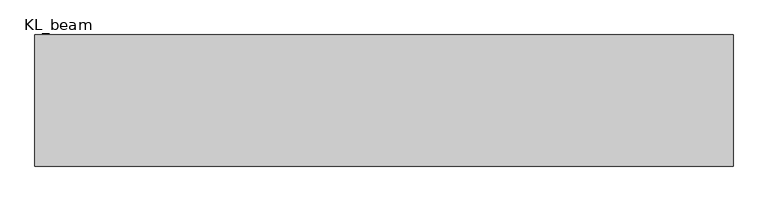
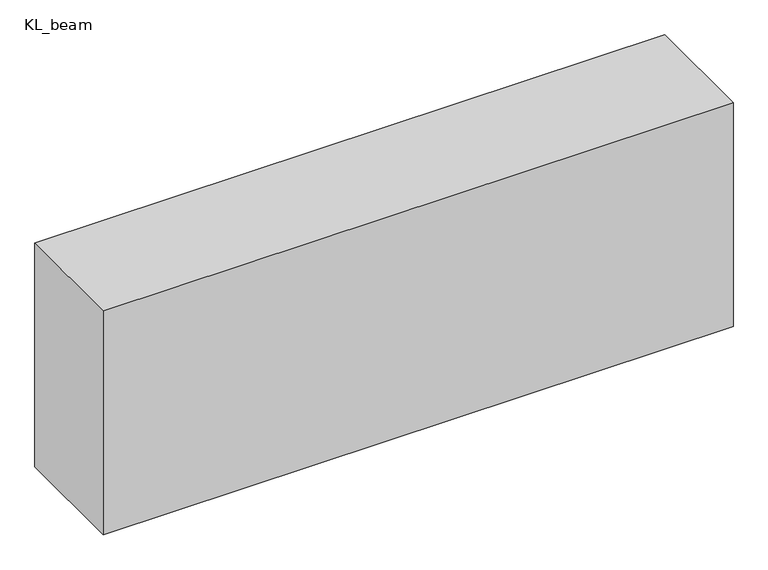
"""IFC4 building model written with IfcOpenShell, lengths in millimetres: beam geometry, 混凝土 - 矩形梁 : KL_beam."""

import ifcopenshell
import ifcopenshell.guid

model = None  # the IFC model being written
_history = None  # IfcOwnerHistory: only IFC2X3 demands one
_inside = {}  # id of a spatial element -> (the spatial element, [elements in it])
_under = {}  # id of a project, library or spatial element -> (it, [spatial elements below it])
_declared = {}  # id of a project -> (the project, [libraries it declares])
_typed = {}  # id of a type object -> (the type object, [elements of that type])
_made_of = {}  # id of a material, layer set ... -> (it, [elements and type objects made of it])


def new_model(schema):
    """Start an empty IFC model of exactly this schema.

    Asked for "IFC4X3", IfcOpenShell would pick the latest addendum, in which some entities
    have other attributes; the version numbers below select the first issue.
    IFC2X3 requires an IfcOwnerHistory on every rooted entity: one is made here for all.
    """
    global model, _history
    if schema == "IFC4X3":
        model = ifcopenshell.file(schema_version=(4, 3, 0, 0))
    else:
        model = ifcopenshell.file(schema=schema)
    _inside.clear()
    _under.clear()
    _declared.clear()
    _typed.clear()
    _made_of.clear()
    _history = None
    if model.schema == "IFC2X3":
        org = make("IfcOrganization", Name="unknown")
        user = make(
            "IfcPersonAndOrganization",
            ThePerson=make("IfcPerson", FamilyName="unknown"),
            TheOrganization=org,
        )
        app = make(
            "IfcApplication",
            ApplicationDeveloper=org,
            Version="unknown",
            ApplicationFullName="unknown",
            ApplicationIdentifier="unknown",
        )
        _history = make(
            "IfcOwnerHistory",
            OwningUser=user,
            OwningApplication=app,
            ChangeAction="ADDED",
            CreationDate=0,
        )
    return model


def make(cls, **values):
    """One entity of the class cls with the attributes given. An attribute that is None is left unset."""
    return model.create_entity(
        cls, **{name: value for name, value in values.items() if value is not None}
    )


def rooted(cls, **values):
    """An entity with a GlobalId (a new one), such as an element, a storey or a relation."""
    return make(cls, GlobalId=ifcopenshell.guid.new(), OwnerHistory=_history, **values)


def si_unit(unit_type, name, prefix=None):
    """IfcSIUnit, for example si_unit("LENGTHUNIT", "METRE", prefix="MILLI")."""
    return make("IfcSIUnit", UnitType=unit_type, Prefix=prefix, Name=name)


def assignment(units):
    """IfcUnitAssignment: the units of a project."""
    return None if units is None else make("IfcUnitAssignment", Units=units)


def point(xyz):
    """IfcCartesianPoint."""
    return None if xyz is None else make("IfcCartesianPoint", Coordinates=xyz)


def direction(xyz):
    """IfcDirection."""
    return None if xyz is None else make("IfcDirection", DirectionRatios=xyz)


def frame(location, z_axis=None, x_axis=None):
    """IfcAxis2Placement3D, a coordinate frame: its origin and axes. An axis left out is left unset."""
    return make(
        "IfcAxis2Placement3D",
        Location=point(location),
        Axis=direction(z_axis),
        RefDirection=direction(x_axis),
    )


def origin():
    """The frame at (0, 0, 0) with its axes left unset."""
    return frame((0.0, 0.0, 0.0))


def place(relative_to, where):
    """IfcLocalPlacement: puts the frame where relative to a parent placement (None: the world)."""
    return make(
        "IfcLocalPlacement", PlacementRelTo=relative_to, RelativePlacement=where
    )


def context(
    kind, dimensions, precision=None, world=None, true_north=None, identifier=None
):
    """IfcGeometricRepresentationContext, for example the 3D "Model" context."""
    return make(
        "IfcGeometricRepresentationContext",
        ContextIdentifier=identifier,
        ContextType=kind,
        CoordinateSpaceDimension=dimensions,
        Precision=precision,
        WorldCoordinateSystem=world,
        TrueNorth=true_north,
    )


def project(units=None, contexts=None):
    """IfcProject with its units and contexts."""
    return rooted(
        "IfcProject",
        Name="project",
        RepresentationContexts=contexts,
        UnitsInContext=assignment(units),
    )


def spatial(cls, under=None, at=None, **own):
    """A site, building, storey or space (cls), placed at a placement, below another one or the project."""
    s = rooted(cls, ObjectPlacement=at, **own)
    if under is not None:
        _under.setdefault(under.id(), (under, []))[1].append(s)
    return s


def polyline(points):
    """IfcPolyline through the points."""
    return make("IfcPolyline", Points=[point(p) for p in points])


def outline(outer, holes=None, kind="AREA"):
    """IfcArbitraryClosedProfileDef: a profile drawn as a closed curve; with holes, ...WithVoids."""
    if holes is None:
        return make("IfcArbitraryClosedProfileDef", ProfileType=kind, OuterCurve=outer)
    return make(
        "IfcArbitraryProfileDefWithVoids",
        ProfileType=kind,
        OuterCurve=outer,
        InnerCurves=holes,
    )


def extrude(swept, where, along, depth):
    """IfcExtrudedAreaSolid: the profile swept, set in the frame where, extruded along a direction by depth."""
    return make(
        "IfcExtrudedAreaSolid",
        SweptArea=swept,
        Position=where,
        ExtrudedDirection=direction(along),
        Depth=depth,
    )


def shape(context_of_items, identifier, shape_type, items):
    """IfcShapeRepresentation: the items that make up one representation, for example the "Body"."""
    return make(
        "IfcShapeRepresentation",
        ContextOfItems=context_of_items,
        RepresentationIdentifier=identifier,
        RepresentationType=shape_type,
        Items=items,
    )


def source(mapping_origin, context_of_items, identifier, shape_type, items):
    """IfcRepresentationMap: a shape defined once, which mapped items show again and again."""
    return make(
        "IfcRepresentationMap",
        MappingOrigin=mapping_origin,
        MappedRepresentation=shape(context_of_items, identifier, shape_type, items),
    )


def transform(
    local_origin,
    x_axis=None,
    y_axis=None,
    z_axis=None,
    scale=None,
    scale2=None,
    scale3=None,
    uniform=True,
):
    """IfcCartesianTransformationOperator3D, or its non-uniform kind. x_axis, y_axis, z_axis: its Axis1, 2, 3."""
    if uniform:
        return make(
            "IfcCartesianTransformationOperator3D",
            Axis1=direction(x_axis),
            Axis2=direction(y_axis),
            LocalOrigin=point(local_origin),
            Scale=scale,
            Axis3=direction(z_axis),
        )
    return make(
        "IfcCartesianTransformationOperator3DnonUniform",
        Axis1=direction(x_axis),
        Axis2=direction(y_axis),
        LocalOrigin=point(local_origin),
        Scale=scale,
        Axis3=direction(z_axis),
        Scale2=scale2,
        Scale3=scale3,
    )


def mapped(mapping_source, mapping_target):
    """IfcMappedItem: shows the shape of a source again, moved by a transform."""
    return make(
        "IfcMappedItem", MappingSource=mapping_source, MappingTarget=mapping_target
    )


def made_of(thing, what):
    """Note that an element or type object is made of a material, layer set ...; save() writes the relation."""
    if what is not None:
        _made_of.setdefault(what.id(), (what, []))[1].append(thing)
    return thing


def element(
    cls,
    number,
    at=None,
    inside=None,
    cuts=None,
    type_object=None,
    material=None,
    context=None,
    identifier="Body",
    shape_type=None,
    held_by="IfcProductDefinitionShape",
    body=None,
    shapes=None,
    **own,
):
    """One element of the class cls, such as IfcWall. Its Tag is "e" and its number.

    at: its placement. inside: the storey or other place that contains it. cuts: it is an
    opening in that element (IfcRelVoidsElement). A single representation is given by context,
    identifier, shape_type and body (its items); several are given by shapes. held_by: the class
    of the entity that holds the representations. save() writes the other relations.
    """
    e = rooted(cls, Tag="e%d" % number, ObjectPlacement=at, **own)
    if body is not None:
        shapes = [shape(context, identifier, shape_type, body)]
    if shapes is not None:
        e.Representation = make(held_by, Representations=shapes)
    if inside is not None:
        _inside.setdefault(inside.id(), (inside, []))[1].append(e)
    if cuts is not None:
        rooted(
            "IfcRelVoidsElement", RelatingBuildingElement=cuts, RelatedOpeningElement=e
        )
    if type_object is not None:
        _typed.setdefault(type_object.id(), (type_object, []))[1].append(e)
    return made_of(e, material)


def aggregate(whole, parts):
    """IfcRelAggregates: a whole, such as a stair, and the parts it consists of."""
    return rooted("IfcRelAggregates", RelatingObject=whole, RelatedObjects=parts)


def save(model, path):
    """Write the relations noted so far, then the file.

    IfcRelAggregates (storeys below a building ...), IfcRelContainedInSpatialStructure (elements
    in a storey), IfcRelDefinesByType, IfcRelAssociatesMaterial and IfcRelDeclares: one each for
    every whole, place, type object, material and project.
    """
    for whole, parts in _under.values():
        aggregate(whole, parts)
    for where, things in _inside.values():
        rooted(
            "IfcRelContainedInSpatialStructure",
            RelatedElements=things,
            RelatingStructure=where,
        )
    for kind, things in _typed.values():
        rooted("IfcRelDefinesByType", RelatedObjects=things, RelatingType=kind)
    for what, things in _made_of.values():
        rooted("IfcRelAssociatesMaterial", RelatedObjects=things, RelatingMaterial=what)
    for by, libraries in _declared.values():
        rooted("IfcRelDeclares", RelatingContext=by, RelatedDefinitions=libraries)
    model.write(path)


def kl_beam_934e2ed8(model_context):
    return source(origin(), model_context, "Body", "SweptSolid", [
        extrude(outline(polyline([(1065.0, 200.0), (1065.0, -200.0), (-1065.0, -200.0), (-1065.0, 200.0), (1065.0, 200.0)])), frame((0.0, 0.0, -400.0), z_axis=(0.0, 0.0, 1.0), x_axis=(1.0, 0.0, 0.0)), (0.0, 0.0, 1.0), 800.0),
    ])


if __name__ == "__main__":
    model = new_model("IFC4")
    model_context = context("Model", 3, world=origin())
    ifc_project = project(units=[si_unit("LENGTHUNIT", "METRE", prefix="MILLI")], contexts=[model_context])
    site = spatial("IfcSite", under=ifc_project)
    building = spatial("IfcBuilding", under=site)
    placement = place(None, origin())
    kl_beam_shape = kl_beam_934e2ed8(model_context)
    element("IfcBeam", 1, ObjectType="混凝土 - 矩形梁 : KL_beam", at=placement, inside=building, context=model_context, shape_type="MappedRepresentation", body=[
        mapped(kl_beam_shape, transform((0.0, 0.0, 0.0), x_axis=(1.0, 0.0, 0.0), y_axis=(0.0, 1.0, 0.0), z_axis=(0.0, 0.0, 1.0))),
    ])
    save(model, "model.ifc")

# Revit data of these elements
# Type "混凝土 - 矩形梁 : KL_beam"
#   Length [instance default] = 1524 mm
#   b = 400 mm
#   h = 800 mm
#   Structural Material [instance default] = 混凝土 - 现场浇注混凝土
#   Assembly Code = ""
# Element 1 (IfcBeam, "混凝土 - 矩形梁 : KL_beam")
#   Structural Material = none
# Materials
#   "混凝土 - 现场浇注混凝土": class "混凝土", colour RGB 192 192 192, transparency 0
